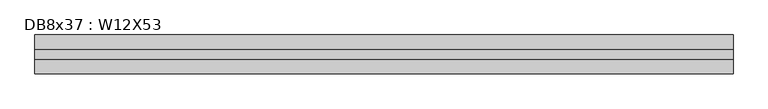
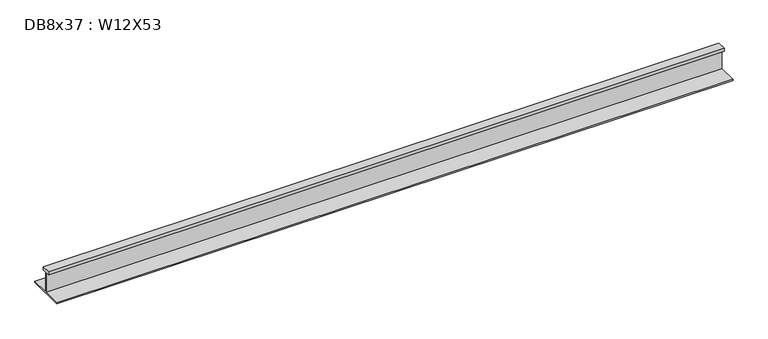
"""IFC4 building model written with IfcOpenShell, lengths in millimetres: beam geometry, DB8x37 : W12X53."""

from ifc_helpers import new_model, si_unit, frame, origin, place, context, project, spatial, polyline, outline, extrude, source, transform, mapped, element, save


def db8x37_w12x53_f22f7946(model_context):
    return source(origin(), model_context, "Body", "SweptSolid", [
        extrude(outline(polyline([(38.1, 145.415), (38.1, 120.015), (2.921, 120.015), (2.921, -48.4505), (152.4, -48.4505), (152.4, -58.1025), (-152.4, -58.1025), (-152.4, -48.4505), (-2.921, -48.4505), (-2.921, 120.015), (-38.1, 120.015), (-38.1, 145.415), (38.1, 145.415)])), frame((-2667.508, 0.0, 0.0), z_axis=(1.0, 0.0, 0.0), x_axis=(0.0, 1.0, 0.0)), (0.0, 0.0, 1.0), 5448.808),
    ])


if __name__ == "__main__":
    model = new_model("IFC4")
    model_context = context("Model", 3, world=origin())
    ifc_project = project(units=[si_unit("LENGTHUNIT", "METRE", prefix="MILLI")], contexts=[model_context])
    site = spatial("IfcSite", under=ifc_project)
    building = spatial("IfcBuilding", under=site)
    placement = place(None, origin())
    db8x37_w12x53_shape = db8x37_w12x53_f22f7946(model_context)
    element("IfcBeam", 1, ObjectType="DB8x37 : W12X53", at=placement, inside=building, context=model_context, shape_type="MappedRepresentation", body=[
        mapped(db8x37_w12x53_shape, transform((0.0, 0.0, 0.0), x_axis=(1.0, 0.0, 0.0), y_axis=(0.0, 1.0, 0.0), z_axis=(0.0, 0.0, 1.0))),
    ])
    save(model, "model.ifc")

# Revit data of these elements
# Type "DB8x37 : W12X53"
#   Assembly Code = "B10"
#   W = 53
#   Length [instance default] = 5' - 0"
#   bf = 0' - 10"
#   d = 1' - 0.1"
#   k = 0' - 1 3/8"
#   k2 = 0' - 0.8"
#   tf = 0' - 0.575"
#   tw = 0' - 0.345"
#   A = 0.108333 SF
#   Structural Material [instance default] = Steel ASTM A992
# Element 1 (IfcBeam, "DB8x37 : W12X53")
#   Materials on its faces: "Steel ASTM A992"
# Materials
#   "Steel ASTM A992": class "Metal", colour RGB 199 199 199, transparency 0, Description = "Structural steel 50ksi", Cost = 0
